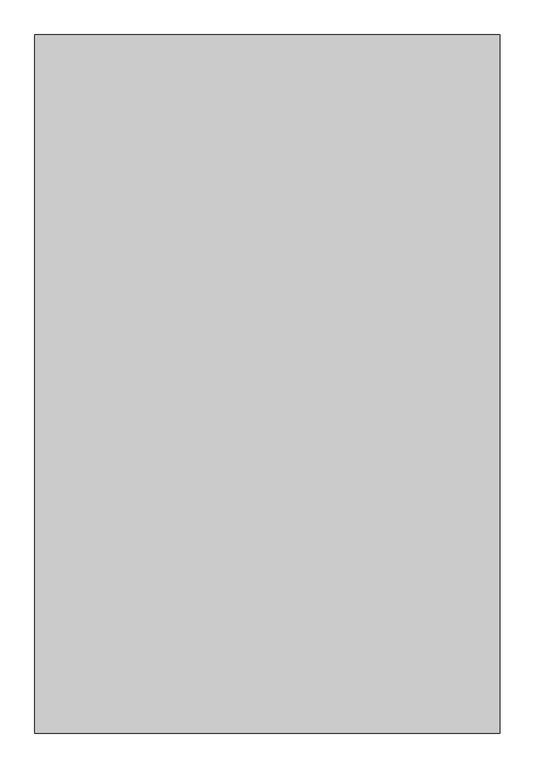
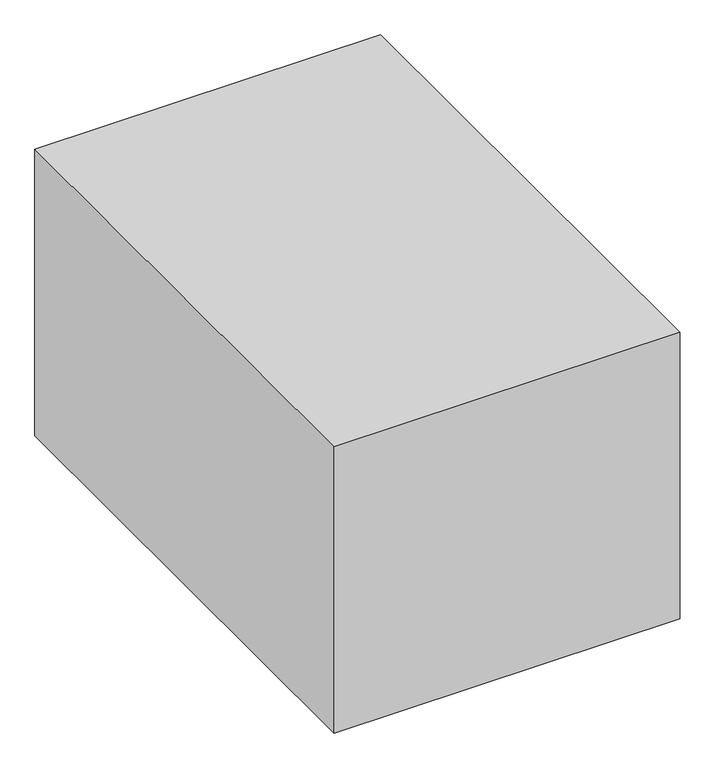
"""IFC4 building model written with IfcOpenShell, lengths in millimetres: proxy geometry, Space Planning Box_hec : Space Planning Box_hec."""

from ifc_helpers import new_model, si_unit, origin, origin_with_axes, place, context, project, spatial, polyline, outline, extrude, source, transform, mapped, element, save


def generic_models_c89eb543(model_context):
    return source(origin(), model_context, "Body", "SweptSolid", [
        extrude(outline(polyline([(2000.0, 3000.0), (2000.0, -3000.0), (-2000.0, -3000.0), (-2000.0, 3000.0), (2000.0, 3000.0)])), origin_with_axes(), (0.0, 0.0, 1.0), 3500.0),
    ])


if __name__ == "__main__":
    model = new_model("IFC4")
    model_context = context("Model", 3, world=origin())
    ifc_project = project(units=[si_unit("LENGTHUNIT", "METRE", prefix="MILLI")], contexts=[model_context])
    site = spatial("IfcSite", under=ifc_project)
    building = spatial("IfcBuilding", under=site)
    placement = place(None, origin())
    generic_models_shape = generic_models_c89eb543(model_context)
    element("IfcBuildingElementProxy", 1, Name="Space Planning Box_hec : Space Planning Box_hec", ObjectType="Space Planning Box_hec : Space Planning Box_hec", at=placement, inside=building, context=model_context, shape_type="MappedRepresentation", body=[
        mapped(generic_models_shape, transform((0.0, 0.0, 0.0), x_axis=(1.0, 0.0, 0.0), y_axis=(0.0, 1.0, 0.0), z_axis=(0.0, 0.0, 1.0))),
    ])
    save(model, "model.ifc")

# Revit data of these elements
# Type "Space Planning Box_hec : Space Planning Box_hec"
#   Type Comments = "..."
#   Room Name [instance default] = "?"
#   Interior Finish [instance default] = ""
#   Exterior Finish [instance default] = ""
#   Department [instance default] = ""
#   Assembly Code = "..."
#   ceiling height [instance default] = 0
#   Width [instance default] = 1524 mm
#   Program Area [instance default] = 0.00 m²
#   Length [instance default] = 1524 mm
#   Height [instance default] = 1524 mm
#   Area [instance default] = 2.32258 m²
#   Fill Color [instance default] = Cyan
#   Default Elevation = 0
# Element 1 (IfcBuildingElementProxy, "Space Planning Box_hec : Space Planning Box_hec")
#   Room Name = "Stairway"
#   Exterior Finish = "N/A..N/A,,EW2..N/A..N/A"
#   Department = "PATHV1"
#   Width = 4000 mm
#   Program Area = 36.00 m²
#   Length = 6000 mm
#   Height = 3500 mm
#   Area = 24.00 m²
#   Fill Color = Green
#   Materials on its faces: "Green"
# Materials
#   "Cyan": class "Generic", colour RGB 0 255 255, transparency 0.2, Cost = 0
#   "Green": class "Generic", colour RGB 0 128 0, transparency 0.2, Cost = 0
